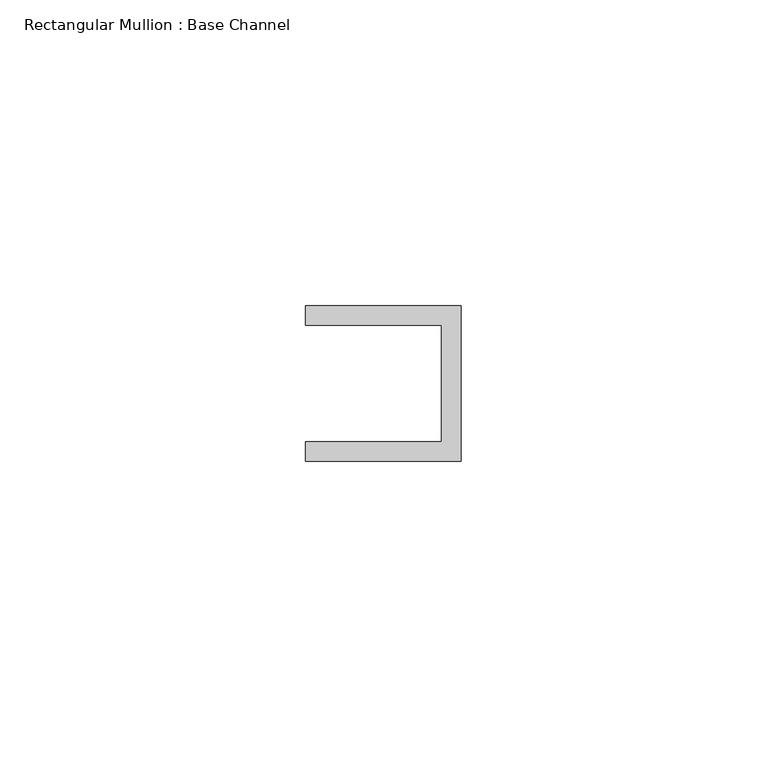
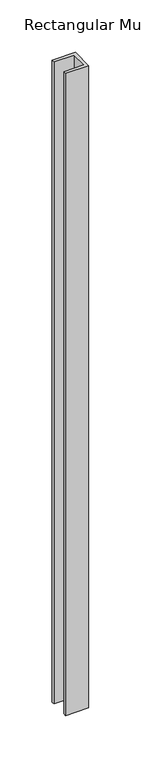
"""IFC4 building model written with IfcOpenShell, lengths in millimetres: member geometry, Rectangular Mullion : Base Channel."""

import ifcopenshell
import ifcopenshell.guid

model = None  # the IFC model being written
_history = None  # IfcOwnerHistory: only IFC2X3 demands one
_inside = {}  # id of a spatial element -> (the spatial element, [elements in it])
_under = {}  # id of a project, library or spatial element -> (it, [spatial elements below it])
_declared = {}  # id of a project -> (the project, [libraries it declares])
_typed = {}  # id of a type object -> (the type object, [elements of that type])
_made_of = {}  # id of a material, layer set ... -> (it, [elements and type objects made of it])


def new_model(schema):
    """Start an empty IFC model of exactly this schema.

    Asked for "IFC4X3", IfcOpenShell would pick the latest addendum, in which some entities
    have other attributes; the version numbers below select the first issue.
    IFC2X3 requires an IfcOwnerHistory on every rooted entity: one is made here for all.
    """
    global model, _history
    if schema == "IFC4X3":
        model = ifcopenshell.file(schema_version=(4, 3, 0, 0))
    else:
        model = ifcopenshell.file(schema=schema)
    _inside.clear()
    _under.clear()
    _declared.clear()
    _typed.clear()
    _made_of.clear()
    _history = None
    if model.schema == "IFC2X3":
        org = make("IfcOrganization", Name="unknown")
        user = make(
            "IfcPersonAndOrganization",
            ThePerson=make("IfcPerson", FamilyName="unknown"),
            TheOrganization=org,
        )
        app = make(
            "IfcApplication",
            ApplicationDeveloper=org,
            Version="unknown",
            ApplicationFullName="unknown",
            ApplicationIdentifier="unknown",
        )
        _history = make(
            "IfcOwnerHistory",
            OwningUser=user,
            OwningApplication=app,
            ChangeAction="ADDED",
            CreationDate=0,
        )
    return model


def make(cls, **values):
    """One entity of the class cls with the attributes given. An attribute that is None is left unset."""
    return model.create_entity(
        cls, **{name: value for name, value in values.items() if value is not None}
    )


def rooted(cls, **values):
    """An entity with a GlobalId (a new one), such as an element, a storey or a relation."""
    return make(cls, GlobalId=ifcopenshell.guid.new(), OwnerHistory=_history, **values)


def si_unit(unit_type, name, prefix=None):
    """IfcSIUnit, for example si_unit("LENGTHUNIT", "METRE", prefix="MILLI")."""
    return make("IfcSIUnit", UnitType=unit_type, Prefix=prefix, Name=name)


def assignment(units):
    """IfcUnitAssignment: the units of a project."""
    return None if units is None else make("IfcUnitAssignment", Units=units)


def point(xyz):
    """IfcCartesianPoint."""
    return None if xyz is None else make("IfcCartesianPoint", Coordinates=xyz)


def direction(xyz):
    """IfcDirection."""
    return None if xyz is None else make("IfcDirection", DirectionRatios=xyz)


def frame(location, z_axis=None, x_axis=None):
    """IfcAxis2Placement3D, a coordinate frame: its origin and axes. An axis left out is left unset."""
    return make(
        "IfcAxis2Placement3D",
        Location=point(location),
        Axis=direction(z_axis),
        RefDirection=direction(x_axis),
    )


def origin():
    """The frame at (0, 0, 0) with its axes left unset."""
    return frame((0.0, 0.0, 0.0))


def place(relative_to, where):
    """IfcLocalPlacement: puts the frame where relative to a parent placement (None: the world)."""
    return make(
        "IfcLocalPlacement", PlacementRelTo=relative_to, RelativePlacement=where
    )


def context(
    kind, dimensions, precision=None, world=None, true_north=None, identifier=None
):
    """IfcGeometricRepresentationContext, for example the 3D "Model" context."""
    return make(
        "IfcGeometricRepresentationContext",
        ContextIdentifier=identifier,
        ContextType=kind,
        CoordinateSpaceDimension=dimensions,
        Precision=precision,
        WorldCoordinateSystem=world,
        TrueNorth=true_north,
    )


def project(units=None, contexts=None):
    """IfcProject with its units and contexts."""
    return rooted(
        "IfcProject",
        Name="project",
        RepresentationContexts=contexts,
        UnitsInContext=assignment(units),
    )


def spatial(cls, under=None, at=None, **own):
    """A site, building, storey or space (cls), placed at a placement, below another one or the project."""
    s = rooted(cls, ObjectPlacement=at, **own)
    if under is not None:
        _under.setdefault(under.id(), (under, []))[1].append(s)
    return s


def polyline(points):
    """IfcPolyline through the points."""
    return make("IfcPolyline", Points=[point(p) for p in points])


def outline(outer, holes=None, kind="AREA"):
    """IfcArbitraryClosedProfileDef: a profile drawn as a closed curve; with holes, ...WithVoids."""
    if holes is None:
        return make("IfcArbitraryClosedProfileDef", ProfileType=kind, OuterCurve=outer)
    return make(
        "IfcArbitraryProfileDefWithVoids",
        ProfileType=kind,
        OuterCurve=outer,
        InnerCurves=holes,
    )


def extrude(swept, where, along, depth):
    """IfcExtrudedAreaSolid: the profile swept, set in the frame where, extruded along a direction by depth."""
    return make(
        "IfcExtrudedAreaSolid",
        SweptArea=swept,
        Position=where,
        ExtrudedDirection=direction(along),
        Depth=depth,
    )


def shape(context_of_items, identifier, shape_type, items):
    """IfcShapeRepresentation: the items that make up one representation, for example the "Body"."""
    return make(
        "IfcShapeRepresentation",
        ContextOfItems=context_of_items,
        RepresentationIdentifier=identifier,
        RepresentationType=shape_type,
        Items=items,
    )


def source(mapping_origin, context_of_items, identifier, shape_type, items):
    """IfcRepresentationMap: a shape defined once, which mapped items show again and again."""
    return make(
        "IfcRepresentationMap",
        MappingOrigin=mapping_origin,
        MappedRepresentation=shape(context_of_items, identifier, shape_type, items),
    )


def transform(
    local_origin,
    x_axis=None,
    y_axis=None,
    z_axis=None,
    scale=None,
    scale2=None,
    scale3=None,
    uniform=True,
):
    """IfcCartesianTransformationOperator3D, or its non-uniform kind. x_axis, y_axis, z_axis: its Axis1, 2, 3."""
    if uniform:
        return make(
            "IfcCartesianTransformationOperator3D",
            Axis1=direction(x_axis),
            Axis2=direction(y_axis),
            LocalOrigin=point(local_origin),
            Scale=scale,
            Axis3=direction(z_axis),
        )
    return make(
        "IfcCartesianTransformationOperator3DnonUniform",
        Axis1=direction(x_axis),
        Axis2=direction(y_axis),
        LocalOrigin=point(local_origin),
        Scale=scale,
        Axis3=direction(z_axis),
        Scale2=scale2,
        Scale3=scale3,
    )


def mapped(mapping_source, mapping_target):
    """IfcMappedItem: shows the shape of a source again, moved by a transform."""
    return make(
        "IfcMappedItem", MappingSource=mapping_source, MappingTarget=mapping_target
    )


def made_of(thing, what):
    """Note that an element or type object is made of a material, layer set ...; save() writes the relation."""
    if what is not None:
        _made_of.setdefault(what.id(), (what, []))[1].append(thing)
    return thing


def element(
    cls,
    number,
    at=None,
    inside=None,
    cuts=None,
    type_object=None,
    material=None,
    context=None,
    identifier="Body",
    shape_type=None,
    held_by="IfcProductDefinitionShape",
    body=None,
    shapes=None,
    **own,
):
    """One element of the class cls, such as IfcWall. Its Tag is "e" and its number.

    at: its placement. inside: the storey or other place that contains it. cuts: it is an
    opening in that element (IfcRelVoidsElement). A single representation is given by context,
    identifier, shape_type and body (its items); several are given by shapes. held_by: the class
    of the entity that holds the representations. save() writes the other relations.
    """
    e = rooted(cls, Tag="e%d" % number, ObjectPlacement=at, **own)
    if body is not None:
        shapes = [shape(context, identifier, shape_type, body)]
    if shapes is not None:
        e.Representation = make(held_by, Representations=shapes)
    if inside is not None:
        _inside.setdefault(inside.id(), (inside, []))[1].append(e)
    if cuts is not None:
        rooted(
            "IfcRelVoidsElement", RelatingBuildingElement=cuts, RelatedOpeningElement=e
        )
    if type_object is not None:
        _typed.setdefault(type_object.id(), (type_object, []))[1].append(e)
    return made_of(e, material)


def aggregate(whole, parts):
    """IfcRelAggregates: a whole, such as a stair, and the parts it consists of."""
    return rooted("IfcRelAggregates", RelatingObject=whole, RelatedObjects=parts)


def save(model, path):
    """Write the relations noted so far, then the file.

    IfcRelAggregates (storeys below a building ...), IfcRelContainedInSpatialStructure (elements
    in a storey), IfcRelDefinesByType, IfcRelAssociatesMaterial and IfcRelDeclares: one each for
    every whole, place, type object, material and project.
    """
    for whole, parts in _under.values():
        aggregate(whole, parts)
    for where, things in _inside.values():
        rooted(
            "IfcRelContainedInSpatialStructure",
            RelatedElements=things,
            RelatingStructure=where,
        )
    for kind, things in _typed.values():
        rooted("IfcRelDefinesByType", RelatedObjects=things, RelatingType=kind)
    for what, things in _made_of.values():
        rooted("IfcRelAssociatesMaterial", RelatedObjects=things, RelatingMaterial=what)
    for by, libraries in _declared.values():
        rooted("IfcRelDeclares", RelatingContext=by, RelatedDefinitions=libraries)
    model.write(path)


def rectangular_mullion_base_channel_118a4787(model_context):
    return source(origin(), model_context, "Body", "SweptSolid", [
        extrude(outline(polyline([(0.0, -12.7), (-25.4, -12.7), (-25.4, -9.525), (-3.175, -9.525), (-3.175, 9.525), (-25.4, 9.525), (-25.4, 12.7), (0.0, 12.7), (0.0, -12.7)])), frame((0.0, 0.0, -747.199643), z_axis=(0.0, 0.0, 1.0), x_axis=(1.0, 0.0, 0.0)), (0.0, 0.0, 1.0), 747.199643),
    ])


if __name__ == "__main__":
    model = new_model("IFC4")
    model_context = context("Model", 3, world=origin())
    ifc_project = project(units=[si_unit("LENGTHUNIT", "METRE", prefix="MILLI")], contexts=[model_context])
    site = spatial("IfcSite", under=ifc_project)
    building = spatial("IfcBuilding", under=site)
    placement = place(None, origin())
    rectangular_mullion_base_channel_shape = rectangular_mullion_base_channel_118a4787(model_context)
    element("IfcMember", 1, ObjectType="Rectangular Mullion : Base Channel", at=placement, inside=building, context=model_context, shape_type="MappedRepresentation", body=[
        mapped(rectangular_mullion_base_channel_shape, transform((0.0, 0.0, 0.0), x_axis=(1.0, 0.0, 0.0), y_axis=(0.0, 1.0, 0.0), z_axis=(0.0, 0.0, 1.0))),
    ])
    save(model, "model.ifc")

# Revit data of these elements
# Type "Rectangular Mullion : Base Channel"
#   built-in parameter 1007322 = 0.0833333 (stored number, unit not read)
#   built-in parameter 1007321 = 0.0416667 (stored number, unit not read)
#   built-in parameter 1007320 = -0.03125 (stored number, unit not read)
# Element 1 (IfcMember, "Rectangular Mullion : Base Channel")
#   Materials on its faces: "ALUM"
# Materials
#   "ALUM": class "Generic", colour RGB 157 157 157, transparency 0, Cost = 0
